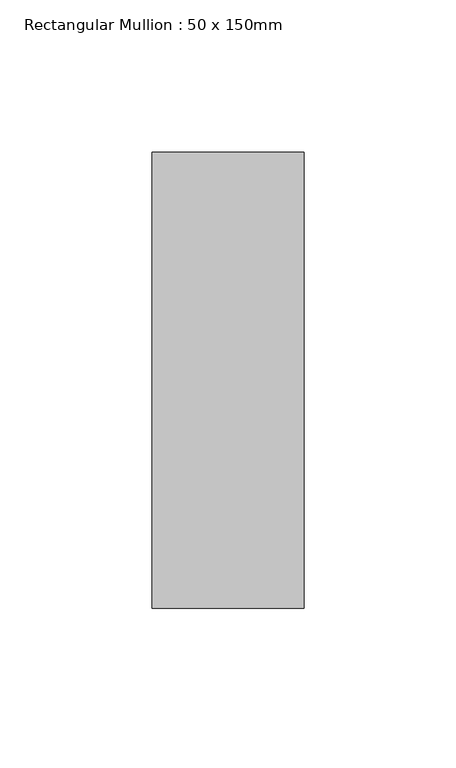
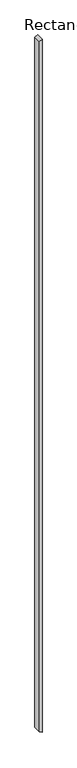
"""IFC4 building model written with IfcOpenShell, lengths in millimetres: member geometry, Rectangular Mullion : 50 x 150mm."""

from ifc_helpers import new_model, si_unit, frame, origin, place, context, project, spatial, polyline, outline, extrude, source, transform, mapped, element, save


def rectangular_mullion_50_x_150mm_7bc3959f(model_context):
    return source(origin(), model_context, "Body", "SweptSolid", [
        extrude(outline(polyline([(0.0, 0.0), (-25.8377402, -50.0), (-13921.2143035, -50.0), (-13951.1008282, 0.0), (0.0, 0.0)])), frame((0.0, -75.0, 0.0), z_axis=(0.0, 1.0, 0.0), x_axis=(0.0, 0.0, 1.0)), (0.0, 0.0, 1.0), 150.0),
    ])


if __name__ == "__main__":
    model = new_model("IFC4")
    model_context = context("Model", 3, world=origin())
    ifc_project = project(units=[si_unit("LENGTHUNIT", "METRE", prefix="MILLI")], contexts=[model_context])
    site = spatial("IfcSite", under=ifc_project)
    building = spatial("IfcBuilding", under=site)
    placement = place(None, origin())
    rectangular_mullion_50_x_150mm_shape = rectangular_mullion_50_x_150mm_7bc3959f(model_context)
    element("IfcMember", 1, ObjectType="Rectangular Mullion : 50 x 150mm", at=placement, inside=building, context=model_context, shape_type="MappedRepresentation", body=[
        mapped(rectangular_mullion_50_x_150mm_shape, transform((0.0, 0.0, 0.0), x_axis=(1.0, 0.0, 0.0), y_axis=(0.0, 1.0, 0.0), z_axis=(0.0, 0.0, 1.0))),
    ])
    save(model, "model.ifc")

# Revit data of these elements
# Type "Rectangular Mullion : 50 x 150mm"
#   built-in parameter 1007304 = 0.492126 (stored number, unit not read)
#   built-in parameter 1007301 = 0.082021 (stored number, unit not read)
#   built-in parameter 1007300 = 0.082021 (stored number, unit not read)
# Element 1 (IfcMember, "Rectangular Mullion : 50 x 150mm")
#   Materials on its faces: "Metal - Aluminium"
# Materials
#   "Metal - Aluminium": class "Metal", colour RGB 247 247 247, transparency 0
